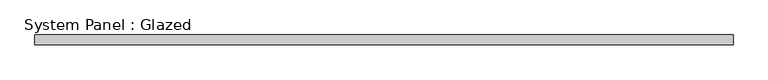
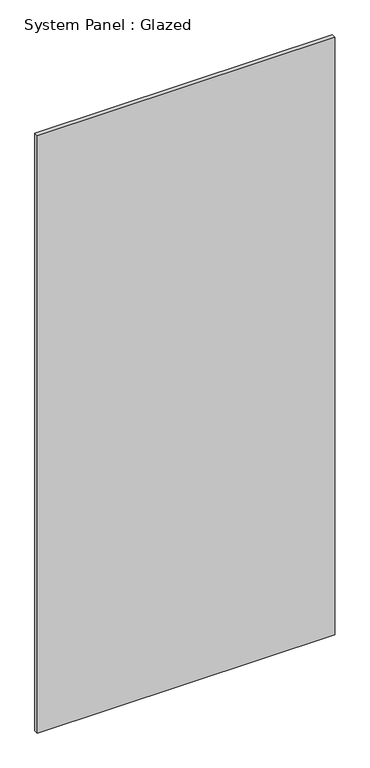
"""IFC4 building model written with IfcOpenShell, lengths in millimetres: plate geometry, System Panel : Glazed."""

import ifcopenshell
import ifcopenshell.guid

model = None  # the IFC model being written
_history = None  # IfcOwnerHistory: only IFC2X3 demands one
_inside = {}  # id of a spatial element -> (the spatial element, [elements in it])
_under = {}  # id of a project, library or spatial element -> (it, [spatial elements below it])
_declared = {}  # id of a project -> (the project, [libraries it declares])
_typed = {}  # id of a type object -> (the type object, [elements of that type])
_made_of = {}  # id of a material, layer set ... -> (it, [elements and type objects made of it])


def new_model(schema):
    """Start an empty IFC model of exactly this schema.

    Asked for "IFC4X3", IfcOpenShell would pick the latest addendum, in which some entities
    have other attributes; the version numbers below select the first issue.
    IFC2X3 requires an IfcOwnerHistory on every rooted entity: one is made here for all.
    """
    global model, _history
    if schema == "IFC4X3":
        model = ifcopenshell.file(schema_version=(4, 3, 0, 0))
    else:
        model = ifcopenshell.file(schema=schema)
    _inside.clear()
    _under.clear()
    _declared.clear()
    _typed.clear()
    _made_of.clear()
    _history = None
    if model.schema == "IFC2X3":
        org = make("IfcOrganization", Name="unknown")
        user = make(
            "IfcPersonAndOrganization",
            ThePerson=make("IfcPerson", FamilyName="unknown"),
            TheOrganization=org,
        )
        app = make(
            "IfcApplication",
            ApplicationDeveloper=org,
            Version="unknown",
            ApplicationFullName="unknown",
            ApplicationIdentifier="unknown",
        )
        _history = make(
            "IfcOwnerHistory",
            OwningUser=user,
            OwningApplication=app,
            ChangeAction="ADDED",
            CreationDate=0,
        )
    return model


def make(cls, **values):
    """One entity of the class cls with the attributes given. An attribute that is None is left unset."""
    return model.create_entity(
        cls, **{name: value for name, value in values.items() if value is not None}
    )


def rooted(cls, **values):
    """An entity with a GlobalId (a new one), such as an element, a storey or a relation."""
    return make(cls, GlobalId=ifcopenshell.guid.new(), OwnerHistory=_history, **values)


def si_unit(unit_type, name, prefix=None):
    """IfcSIUnit, for example si_unit("LENGTHUNIT", "METRE", prefix="MILLI")."""
    return make("IfcSIUnit", UnitType=unit_type, Prefix=prefix, Name=name)


def assignment(units):
    """IfcUnitAssignment: the units of a project."""
    return None if units is None else make("IfcUnitAssignment", Units=units)


def point(xyz):
    """IfcCartesianPoint."""
    return None if xyz is None else make("IfcCartesianPoint", Coordinates=xyz)


def direction(xyz):
    """IfcDirection."""
    return None if xyz is None else make("IfcDirection", DirectionRatios=xyz)


def frame(location, z_axis=None, x_axis=None):
    """IfcAxis2Placement3D, a coordinate frame: its origin and axes. An axis left out is left unset."""
    return make(
        "IfcAxis2Placement3D",
        Location=point(location),
        Axis=direction(z_axis),
        RefDirection=direction(x_axis),
    )


def origin():
    """The frame at (0, 0, 0) with its axes left unset."""
    return frame((0.0, 0.0, 0.0))


def origin_with_axes():
    """The frame at (0, 0, 0) with the z axis (0, 0, 1) and the x axis (1, 0, 0) written out."""
    return frame((0.0, 0.0, 0.0), z_axis=(0.0, 0.0, 1.0), x_axis=(1.0, 0.0, 0.0))


def place(relative_to, where):
    """IfcLocalPlacement: puts the frame where relative to a parent placement (None: the world)."""
    return make(
        "IfcLocalPlacement", PlacementRelTo=relative_to, RelativePlacement=where
    )


def context(
    kind, dimensions, precision=None, world=None, true_north=None, identifier=None
):
    """IfcGeometricRepresentationContext, for example the 3D "Model" context."""
    return make(
        "IfcGeometricRepresentationContext",
        ContextIdentifier=identifier,
        ContextType=kind,
        CoordinateSpaceDimension=dimensions,
        Precision=precision,
        WorldCoordinateSystem=world,
        TrueNorth=true_north,
    )


def project(units=None, contexts=None):
    """IfcProject with its units and contexts."""
    return rooted(
        "IfcProject",
        Name="project",
        RepresentationContexts=contexts,
        UnitsInContext=assignment(units),
    )


def spatial(cls, under=None, at=None, **own):
    """A site, building, storey or space (cls), placed at a placement, below another one or the project."""
    s = rooted(cls, ObjectPlacement=at, **own)
    if under is not None:
        _under.setdefault(under.id(), (under, []))[1].append(s)
    return s


def polyline(points):
    """IfcPolyline through the points."""
    return make("IfcPolyline", Points=[point(p) for p in points])


def outline(outer, holes=None, kind="AREA"):
    """IfcArbitraryClosedProfileDef: a profile drawn as a closed curve; with holes, ...WithVoids."""
    if holes is None:
        return make("IfcArbitraryClosedProfileDef", ProfileType=kind, OuterCurve=outer)
    return make(
        "IfcArbitraryProfileDefWithVoids",
        ProfileType=kind,
        OuterCurve=outer,
        InnerCurves=holes,
    )


def extrude(swept, where, along, depth):
    """IfcExtrudedAreaSolid: the profile swept, set in the frame where, extruded along a direction by depth."""
    return make(
        "IfcExtrudedAreaSolid",
        SweptArea=swept,
        Position=where,
        ExtrudedDirection=direction(along),
        Depth=depth,
    )


def shape(context_of_items, identifier, shape_type, items):
    """IfcShapeRepresentation: the items that make up one representation, for example the "Body"."""
    return make(
        "IfcShapeRepresentation",
        ContextOfItems=context_of_items,
        RepresentationIdentifier=identifier,
        RepresentationType=shape_type,
        Items=items,
    )


def source(mapping_origin, context_of_items, identifier, shape_type, items):
    """IfcRepresentationMap: a shape defined once, which mapped items show again and again."""
    return make(
        "IfcRepresentationMap",
        MappingOrigin=mapping_origin,
        MappedRepresentation=shape(context_of_items, identifier, shape_type, items),
    )


def transform(
    local_origin,
    x_axis=None,
    y_axis=None,
    z_axis=None,
    scale=None,
    scale2=None,
    scale3=None,
    uniform=True,
):
    """IfcCartesianTransformationOperator3D, or its non-uniform kind. x_axis, y_axis, z_axis: its Axis1, 2, 3."""
    if uniform:
        return make(
            "IfcCartesianTransformationOperator3D",
            Axis1=direction(x_axis),
            Axis2=direction(y_axis),
            LocalOrigin=point(local_origin),
            Scale=scale,
            Axis3=direction(z_axis),
        )
    return make(
        "IfcCartesianTransformationOperator3DnonUniform",
        Axis1=direction(x_axis),
        Axis2=direction(y_axis),
        LocalOrigin=point(local_origin),
        Scale=scale,
        Axis3=direction(z_axis),
        Scale2=scale2,
        Scale3=scale3,
    )


def mapped(mapping_source, mapping_target):
    """IfcMappedItem: shows the shape of a source again, moved by a transform."""
    return make(
        "IfcMappedItem", MappingSource=mapping_source, MappingTarget=mapping_target
    )


def made_of(thing, what):
    """Note that an element or type object is made of a material, layer set ...; save() writes the relation."""
    if what is not None:
        _made_of.setdefault(what.id(), (what, []))[1].append(thing)
    return thing


def element(
    cls,
    number,
    at=None,
    inside=None,
    cuts=None,
    type_object=None,
    material=None,
    context=None,
    identifier="Body",
    shape_type=None,
    held_by="IfcProductDefinitionShape",
    body=None,
    shapes=None,
    **own,
):
    """One element of the class cls, such as IfcWall. Its Tag is "e" and its number.

    at: its placement. inside: the storey or other place that contains it. cuts: it is an
    opening in that element (IfcRelVoidsElement). A single representation is given by context,
    identifier, shape_type and body (its items); several are given by shapes. held_by: the class
    of the entity that holds the representations. save() writes the other relations.
    """
    e = rooted(cls, Tag="e%d" % number, ObjectPlacement=at, **own)
    if body is not None:
        shapes = [shape(context, identifier, shape_type, body)]
    if shapes is not None:
        e.Representation = make(held_by, Representations=shapes)
    if inside is not None:
        _inside.setdefault(inside.id(), (inside, []))[1].append(e)
    if cuts is not None:
        rooted(
            "IfcRelVoidsElement", RelatingBuildingElement=cuts, RelatedOpeningElement=e
        )
    if type_object is not None:
        _typed.setdefault(type_object.id(), (type_object, []))[1].append(e)
    return made_of(e, material)


def aggregate(whole, parts):
    """IfcRelAggregates: a whole, such as a stair, and the parts it consists of."""
    return rooted("IfcRelAggregates", RelatingObject=whole, RelatedObjects=parts)


def save(model, path):
    """Write the relations noted so far, then the file.

    IfcRelAggregates (storeys below a building ...), IfcRelContainedInSpatialStructure (elements
    in a storey), IfcRelDefinesByType, IfcRelAssociatesMaterial and IfcRelDeclares: one each for
    every whole, place, type object, material and project.
    """
    for whole, parts in _under.values():
        aggregate(whole, parts)
    for where, things in _inside.values():
        rooted(
            "IfcRelContainedInSpatialStructure",
            RelatedElements=things,
            RelatingStructure=where,
        )
    for kind, things in _typed.values():
        rooted("IfcRelDefinesByType", RelatedObjects=things, RelatingType=kind)
    for what, things in _made_of.values():
        rooted("IfcRelAssociatesMaterial", RelatedObjects=things, RelatingMaterial=what)
    for by, libraries in _declared.values():
        rooted("IfcRelDeclares", RelatingContext=by, RelatedDefinitions=libraries)
    model.write(path)


def system_panel_glazed_e1325fc6(model_context):
    return source(origin(), model_context, "Body", "SweptSolid", [
        extrude(outline(polyline([(894.9999998, 24.5), (-894.9999998, 24.5), (-894.9999998, 49.5), (894.9999998, 49.5), (894.9999998, 24.5)])), origin_with_axes(), (0.0, 0.0, 1.0), 3800.0),
    ])


if __name__ == "__main__":
    model = new_model("IFC4")
    model_context = context("Model", 3, world=origin())
    ifc_project = project(units=[si_unit("LENGTHUNIT", "METRE", prefix="MILLI")], contexts=[model_context])
    site = spatial("IfcSite", under=ifc_project)
    building = spatial("IfcBuilding", under=site)
    placement = place(None, origin())
    system_panel_glazed_shape = system_panel_glazed_e1325fc6(model_context)
    element("IfcPlate", 1, ObjectType="System Panel : Glazed", at=placement, inside=building, context=model_context, shape_type="MappedRepresentation", body=[
        mapped(system_panel_glazed_shape, transform((0.0, 0.0, 0.0), x_axis=(1.0, 0.0, 0.0), y_axis=(0.0, 1.0, 0.0), z_axis=(0.0, 0.0, 1.0))),
    ])
    save(model, "model.ifc")

# Revit data of these elements
# Type "System Panel : Glazed"
#   Construction Type Id = "GSP4R"
#   Analytic Construction = "1/8 in Pilkington single glazing"
#   Visual Light Transmittance = 0.9
#   Solar Heat Gain Coefficient = 0.86
#   Heat Transfer Coefficient (U) = 6.7069 W/(m²·K)
#   Define Thermal Properties by = 1
# Element 1 (IfcPlate, "System Panel : Glazed")
#   Materials on its faces: "Glass"
# Materials
#   "Glass": class "Glass", colour RGB 0 128 192, transparency 0.9, Description = "Soda Lime Glass", Cost = 0
